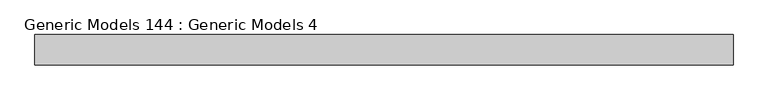
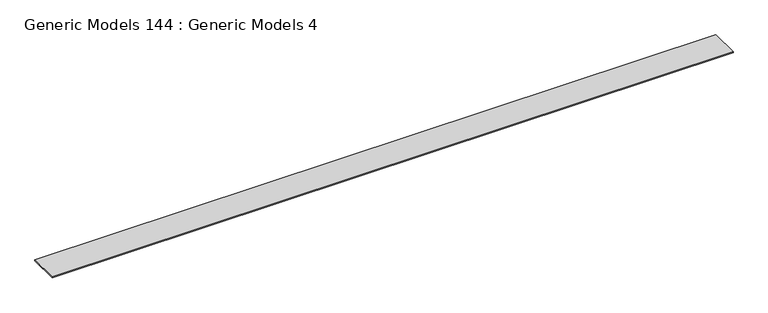
"""IFC4 building model written with IfcOpenShell, lengths in millimetres: proxy geometry, Generic Models 144 : Generic Models 4."""

from ifc_helpers import new_model, si_unit, frame, origin, place, context, project, spatial, polyline, outline, extrude, source, transform, mapped, element, save


def generic_models_144_generic_models_4_d644e738(model_context):
    return source(origin(), model_context, "Body", "SweptSolid", [
        extrude(outline(polyline([(20644.6159513, 7212.6867903), (20644.6159513, 7761.1754549), (33192.2159513, 7761.1754549), (33192.2159513, 7212.6867903), (20644.6159513, 7212.6867903)])), frame((0.0, 0.0, 124030.3826265), z_axis=(0.0, 0.0, 1.0), x_axis=(1.0, 0.0, 0.0)), (0.0, 0.0, 1.0), 17.4625),
    ])


if __name__ == "__main__":
    model = new_model("IFC4")
    model_context = context("Model", 3, world=origin())
    ifc_project = project(units=[si_unit("LENGTHUNIT", "METRE", prefix="MILLI")], contexts=[model_context])
    site = spatial("IfcSite", under=ifc_project)
    building = spatial("IfcBuilding", under=site)
    placement = place(None, origin())
    generic_models_144_generic_models_4_shape = generic_models_144_generic_models_4_d644e738(model_context)
    element("IfcBuildingElementProxy", 1, Name="Generic Models 144 : Generic Models 4", ObjectType="Generic Models 144 : Generic Models 4", at=placement, inside=building, context=model_context, shape_type="MappedRepresentation", body=[
        mapped(generic_models_144_generic_models_4_shape, transform((0.0, 0.0, 0.0), x_axis=(1.0, 0.0, 0.0), y_axis=(0.0, 1.0, 0.0), z_axis=(0.0, 0.0, 1.0))),
    ])
    save(model, "model.ifc")

# Revit data of these elements
# Element 1 (IfcBuildingElementProxy, "Generic Models 144 : Generic Models 4")
#   Materials on its faces: "_3/4\" TREATED CDX PLYWOOD"
# Materials
#   "_3/4\" TREATED CDX PLYWOOD": class "Generic", colour RGB 98 75 74, transparency 0, Cost = 0
